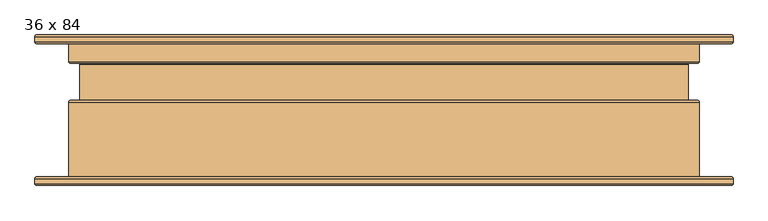
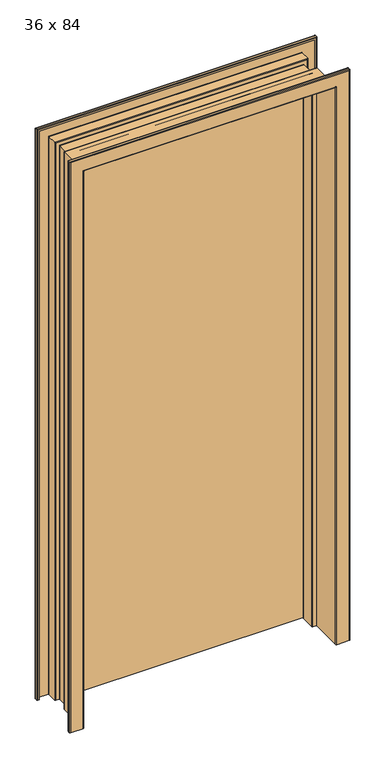
"""IFC4 building model written with IfcOpenShell, lengths in millimetres: door geometry, Door-Dunbarton_Doors-Hollow_Metal_Core : 36 x 84."""

from ifc_helpers import new_model, si_unit, frame, origin, origin_with_axes, place, context, project, spatial, polyline, circle_curve, ellipse_curve, outline, extrude, source, transform, mapped, element, save
from ifc_brep_helpers import plane_surface, cylinder_surface, revolved_surface, advanced_brep


def door_36_x_84_b8b41eee(model_context):
    return source(origin(), model_context, "Body", "SolidModel", [
        advanced_brep(
        [(-505.42825, -96.901, 0.0), (-500.0625, -96.901, 0.0), (-500.0625, -98.45675, 0.0), (-505.42825, -98.45675, 0.0), (-506.44425, -99.47275, 0.0), (-506.44425, -106.9975, 0.0), (-505.42825, -108.0135, 0.0), (-459.77175, -108.0135, 0.0), (-458.75575, -106.9975, 0.0), (-458.75575, 11.65225, 0.0), (-456.184, 14.224, 0.0), (-443.89675, 14.224, 0.0), (-442.88075, 15.24, 0.0), (-442.88075, 67.0306, 0.0), (-443.89675, 68.0466, 0.0), (-456.184, 68.0466, 0.0), (-458.75575, 70.61835, 0.0), (-458.75575, 106.934, 0.0), (-459.77175, 107.95, 0.0), (-505.42825, 107.95, 0.0), (-506.44425, 106.934, 0.0), (-506.44425, 99.40925, 0.0), (-505.42825, 98.39325, 0.0), (-500.0625, 98.39325, 0.0), (-500.0625, 96.8375, 0.0), (-505.42825, 96.8375, 0.0), (-508.0, 99.40925, 0.0), (-508.0, 106.934, 0.0), (-505.42825, 109.50575, 0.0), (-459.77175, 109.50575, 0.0), (-457.2, 106.934, 0.0), (-457.2, 70.61835, 0.0), (-456.184, 69.60235, 0.0), (-443.89675, 69.60235, 0.0), (-441.325, 67.0306, 0.0), (-441.325, 15.24, 0.0), (-443.89675, 12.66825, 0.0), (-456.184, 12.66825, 0.0), (-457.2, 11.65225, 0.0), (-457.2, -106.9975, 0.0), (-459.77175, -109.56925, 0.0), (-505.42825, -109.56925, 0.0), (-508.0, -106.9975, 0.0), (-508.0, -99.47275, 0.0), (-508.0, -99.47275, 2184.4), (-505.42825, -96.901, 2181.82825), (-508.0, -106.9975, 2184.4), (-505.42825, -109.56925, 2181.82825), (-459.77175, -109.56925, 2136.17175), (459.77175, -109.56925, 2136.17175), (459.77175, -109.56925, 0.0), (505.42825, -109.56925, 0.0), (505.42825, -109.56925, 2181.82825), (-457.2, -106.9975, 2133.6), (-457.2, 11.65225, 2133.6), (-456.184, 12.66825, 2132.584), (-443.89675, 12.66825, 2120.29675), (443.89675, 12.66825, 2120.29675), (443.89675, 12.66825, 0.0), (456.184, 12.66825, 0.0), (456.184, 12.66825, 2132.584), (-441.325, 15.24, 2117.725), (-441.325, 67.0306, 2117.725), (-443.89675, 69.60235, 2120.29675), (-456.184, 69.60235, 2132.584), (456.184, 69.60235, 2132.584), (456.184, 69.60235, 0.0), (443.89675, 69.60235, 0.0), (443.89675, 69.60235, 2120.29675), (-457.2, 70.61835, 2133.6), (-457.2, 106.934, 2133.6), (-459.77175, 109.50575, 2136.17175), (-505.42825, 109.50575, 2181.82825), (505.42825, 109.50575, 2181.82825), (505.42825, 109.50575, 0.0), (459.77175, 109.50575, 0.0), (459.77175, 109.50575, 2136.17175), (-508.0, 106.934, 2184.4), (-508.0, 99.40925, 2184.4), (-505.42825, 96.8375, 2181.82825), (-500.0625, 96.8375, 2176.4625), (500.0625, 96.8375, 2176.4625), (500.0625, 96.8375, 0.0), (505.42825, 96.8375, 0.0), (505.42825, 96.8375, 2181.82825), (-500.0625, 98.39325, 2176.4625), (-505.42825, 98.39325, 2181.82825), (505.42825, 98.39325, 2181.82825), (505.42825, 98.39325, 0.0), (500.0625, 98.39325, 0.0), (500.0625, 98.39325, 2176.4625), (-506.44425, 99.40925, 2182.84425), (-506.44425, 106.934, 2182.84425), (-505.42825, 107.95, 2181.82825), (-459.77175, 107.95, 2136.17175), (459.77175, 107.95, 2136.17175), (459.77175, 107.95, 0.0), (505.42825, 107.95, 0.0), (505.42825, 107.95, 2181.82825), (-458.75575, 106.934, 2135.15575), (-458.75575, 70.61835, 2135.15575), (-456.184, 68.0466, 2132.584), (-443.89675, 68.0466, 2120.29675), (443.89675, 68.0466, 2120.29675), (443.89675, 68.0466, 0.0), (456.184, 68.0466, 0.0), (456.184, 68.0466, 2132.584), (-442.88075, 67.0306, 2119.28075), (-442.88075, 15.24, 2119.28075), (-443.89675, 14.224, 2120.29675), (-456.184, 14.224, 2132.584), (456.184, 14.224, 2132.584), (456.184, 14.224, 0.0), (443.89675, 14.224, 0.0), (443.89675, 14.224, 2120.29675), (-458.75575, 11.65225, 2135.15575), (-458.75575, -106.9975, 2135.15575), (-459.77175, -108.0135, 2136.17175), (-505.42825, -108.0135, 2181.82825), (505.42825, -108.0135, 2181.82825), (505.42825, -108.0135, 0.0), (459.77175, -108.0135, 0.0), (459.77175, -108.0135, 2136.17175), (-506.44425, -106.9975, 2182.84425), (-506.44425, -99.47275, 2182.84425), (-505.42825, -98.45675, 2181.82825), (-500.0625, -98.45675, 2176.4625), (500.0625, -98.45675, 2176.4625), (500.0625, -98.45675, 0.0), (505.42825, -98.45675, 0.0), (505.42825, -98.45675, 2181.82825), (-500.0625, -96.901, 2176.4625), (505.42825, -96.901, 2181.82825), (505.42825, -96.901, 0.0), (500.0625, -96.901, 0.0), (500.0625, -96.901, 2176.4625), (508.0, -99.47275, 2184.4), (508.0, -106.9975, 2184.4), (457.2, -106.9975, 2133.6), (457.2, 11.65225, 2133.6), (441.325, 15.24, 2117.725), (441.325, 67.0306, 2117.725), (457.2, 70.61835, 2133.6), (457.2, 106.934, 2133.6), (508.0, 106.934, 2184.4), (508.0, 99.40925, 2184.4), (506.44425, 99.40925, 2182.84425), (506.44425, 106.934, 2182.84425), (458.75575, 106.934, 2135.15575), (458.75575, 70.61835, 2135.15575), (442.88075, 67.0306, 2119.28075), (442.88075, 15.24, 2119.28075), (458.75575, 11.65225, 2135.15575), (458.75575, -106.9975, 2135.15575), (506.44425, -106.9975, 2182.84425), (506.44425, -99.47275, 2182.84425), (508.0, -99.47275, 0.0), (508.0, -106.9975, 0.0), (457.2, -106.9975, 0.0), (457.2, 11.65225, 0.0), (441.325, 15.24, 0.0), (441.325, 67.0306, 0.0), (457.2, 70.61835, 0.0), (457.2, 106.934, 0.0), (508.0, 106.934, 0.0), (508.0, 99.40925, 0.0), (506.44425, 99.40925, 0.0), (506.44425, 106.934, 0.0), (458.75575, 106.934, 0.0), (458.75575, 70.61835, 0.0), (442.88075, 67.0306, 0.0), (442.88075, 15.24, 0.0), (458.75575, 11.65225, 0.0), (458.75575, -106.9975, 0.0), (506.44425, -106.9975, 0.0), (506.44425, -99.47275, 0.0)],
        [
            (0, 1),
            (1, 2),
            (2, 3),
            (3, 4, circle_curve(frame((-505.42825, -99.47275, 0.0), z_axis=(0.0, 0.0, 1.0), x_axis=(0.0, 1.0, 0.0)), 1.016)),
            (4, 5),
            (5, 6, circle_curve(frame((-505.42825, -106.9975, 0.0), z_axis=(0.0, 0.0, 1.0), x_axis=(0.0, 1.0, 0.0)), 1.016)),
            (6, 7),
            (7, 8, circle_curve(frame((-459.77175, -106.9975, 0.0), z_axis=(0.0, 0.0, 1.0), x_axis=(0.0, 1.0, 0.0)), 1.016)),
            (8, 9),
            (9, 10, circle_curve(frame((-456.184, 11.65225, 0.0), z_axis=(0.0, 0.0, -1.0), x_axis=(0.0, 1.0, 0.0)), 2.57175)),
            (10, 11),
            (11, 12, circle_curve(frame((-443.89675, 15.24, 0.0), z_axis=(0.0, 0.0, 1.0), x_axis=(0.0, 1.0, 0.0)), 1.016)),
            (12, 13),
            (13, 14, circle_curve(frame((-443.89675, 67.0306, 0.0), z_axis=(0.0, 0.0, 1.0), x_axis=(0.0, 1.0, 0.0)), 1.016)),
            (14, 15),
            (15, 16, circle_curve(frame((-456.184, 70.61835, 0.0), z_axis=(0.0, 0.0, -1.0), x_axis=(0.0, 1.0, 0.0)), 2.57175)),
            (16, 17),
            (17, 18, circle_curve(frame((-459.77175, 106.934, 0.0), z_axis=(0.0, 0.0, 1.0), x_axis=(0.0, 1.0, 0.0)), 1.016)),
            (18, 19),
            (19, 20, circle_curve(frame((-505.42825, 106.934, 0.0), z_axis=(0.0, 0.0, 1.0), x_axis=(0.0, 1.0, 0.0)), 1.016)),
            (20, 21),
            (21, 22, circle_curve(frame((-505.42825, 99.40925, 0.0), z_axis=(0.0, 0.0, 1.0), x_axis=(0.0, 1.0, 0.0)), 1.016)),
            (22, 23),
            (23, 24),
            (24, 25),
            (25, 26, circle_curve(frame((-505.42825, 99.40925, 0.0), z_axis=(0.0, 0.0, -1.0), x_axis=(0.0, 1.0, 0.0)), 2.57175)),
            (26, 27),
            (27, 28, circle_curve(frame((-505.42825, 106.934, 0.0), z_axis=(0.0, 0.0, -1.0), x_axis=(0.0, 1.0, 0.0)), 2.57175)),
            (28, 29),
            (29, 30, circle_curve(frame((-459.77175, 106.934, 0.0), z_axis=(0.0, 0.0, -1.0), x_axis=(0.0, 1.0, 0.0)), 2.57175)),
            (30, 31),
            (31, 32, circle_curve(frame((-456.184, 70.61835, 0.0), z_axis=(0.0, 0.0, 1.0), x_axis=(0.0, 1.0, 0.0)), 1.016)),
            (32, 33),
            (33, 34, circle_curve(frame((-443.89675, 67.0306, 0.0), z_axis=(0.0, 0.0, -1.0), x_axis=(0.0, 1.0, 0.0)), 2.57175)),
            (34, 35),
            (35, 36, circle_curve(frame((-443.89675, 15.24, 0.0), z_axis=(0.0, 0.0, -1.0), x_axis=(0.0, 1.0, 0.0)), 2.57175)),
            (36, 37),
            (37, 38, circle_curve(frame((-456.184, 11.65225, 0.0), z_axis=(0.0, 0.0, 1.0), x_axis=(0.0, 1.0, 0.0)), 1.016)),
            (38, 39),
            (39, 40, circle_curve(frame((-459.77175, -106.9975, 0.0), z_axis=(0.0, 0.0, -1.0), x_axis=(0.0, 1.0, 0.0)), 2.57175)),
            (40, 41),
            (41, 42, circle_curve(frame((-505.42825, -106.9975, 0.0), z_axis=(0.0, 0.0, -1.0), x_axis=(0.0, 1.0, 0.0)), 2.57175)),
            (42, 43),
            (43, 0, circle_curve(frame((-505.42825, -99.47275, 0.0), z_axis=(0.0, 0.0, -1.0), x_axis=(0.0, 1.0, 0.0)), 2.57175)),
            (43, 44),
            (44, 45, ellipse_curve(frame((-505.42825, -99.47275, 2181.82825), z_axis=(-0.7071067811865475, 0.0, -0.7071067811865475), x_axis=(0.7071067811865474, 0.0, -0.7071067811865476)), 3.6370037, 2.57175)),
            (45, 0),
            (42, 46),
            (46, 44),
            (41, 47),
            (47, 46, ellipse_curve(frame((-505.42825, -106.9975, 2181.82825), z_axis=(-0.7071067811865475, 0.0, -0.7071067811865475), x_axis=(0.7071067811865474, 0.0, -0.7071067811865476)), 3.6370037, 2.57175)),
            (40, 48),
            (48, 49),
            (49, 50),
            (50, 51),
            (51, 52),
            (52, 47),
            (39, 53),
            (53, 48, ellipse_curve(frame((-459.77175, -106.9975, 2136.17175), z_axis=(-0.7071067811865475, 0.0, -0.7071067811865475), x_axis=(0.7071067811865474, 0.0, -0.7071067811865476)), 3.6370037, 2.57175)),
            (38, 54),
            (54, 53),
            (37, 55),
            (55, 54, ellipse_curve(frame((-456.184, 11.65225, 2132.584), z_axis=(0.7071067811865475, 0.0, 0.7071067811865475), x_axis=(-0.7071067811865474, 0.0, 0.7071067811865476)), 1.436841, 1.016)),
            (36, 56),
            (56, 57),
            (57, 58),
            (58, 59),
            (59, 60),
            (60, 55),
            (35, 61),
            (61, 56, ellipse_curve(frame((-443.89675, 15.24, 2120.29675), z_axis=(-0.7071067811865475, 0.0, -0.7071067811865475), x_axis=(0.7071067811865474, 0.0, -0.7071067811865476)), 3.6370037, 2.57175)),
            (34, 62),
            (62, 61),
            (33, 63),
            (63, 62, ellipse_curve(frame((-443.89675, 67.0306, 2120.29675), z_axis=(-0.7071067811865475, 0.0, -0.7071067811865475), x_axis=(0.7071067811865474, 0.0, -0.7071067811865476)), 3.6370037, 2.57175)),
            (32, 64),
            (64, 65),
            (65, 66),
            (66, 67),
            (67, 68),
            (68, 63),
            (31, 69),
            (69, 64, ellipse_curve(frame((-456.184, 70.61835, 2132.584), z_axis=(0.7071067811865475, 0.0, 0.7071067811865475), x_axis=(-0.7071067811865474, 0.0, 0.7071067811865476)), 1.436841, 1.016)),
            (30, 70),
            (70, 69),
            (29, 71),
            (71, 70, ellipse_curve(frame((-459.77175, 106.934, 2136.17175), z_axis=(-0.7071067811865475, 0.0, -0.7071067811865475), x_axis=(0.7071067811865474, 0.0, -0.7071067811865476)), 3.6370037, 2.57175)),
            (28, 72),
            (72, 73),
            (73, 74),
            (74, 75),
            (75, 76),
            (76, 71),
            (27, 77),
            (77, 72, ellipse_curve(frame((-505.42825, 106.934, 2181.82825), z_axis=(-0.7071067811865475, 0.0, -0.7071067811865475), x_axis=(0.7071067811865474, 0.0, -0.7071067811865476)), 3.6370037, 2.57175)),
            (26, 78),
            (78, 77),
            (25, 79),
            (79, 78, ellipse_curve(frame((-505.42825, 99.40925, 2181.82825), z_axis=(-0.7071067811865475, 0.0, -0.7071067811865475), x_axis=(0.7071067811865474, 0.0, -0.7071067811865476)), 3.6370037, 2.57175)),
            (24, 80),
            (80, 81),
            (81, 82),
            (82, 83),
            (83, 84),
            (84, 79),
            (23, 85),
            (85, 80),
            (22, 86),
            (86, 87),
            (87, 88),
            (88, 89),
            (89, 90),
            (90, 85),
            (21, 91),
            (91, 86, ellipse_curve(frame((-505.42825, 99.40925, 2181.82825), z_axis=(0.7071067811865475, 0.0, 0.7071067811865475), x_axis=(-0.7071067811865474, 0.0, 0.7071067811865476)), 1.436841, 1.016)),
            (20, 92),
            (92, 91),
            (19, 93),
            (93, 92, ellipse_curve(frame((-505.42825, 106.934, 2181.82825), z_axis=(0.7071067811865475, 0.0, 0.7071067811865475), x_axis=(-0.7071067811865474, 0.0, 0.7071067811865476)), 1.436841, 1.016)),
            (18, 94),
            (94, 95),
            (95, 96),
            (96, 97),
            (97, 98),
            (98, 93),
            (17, 99),
            (99, 94, ellipse_curve(frame((-459.77175, 106.934, 2136.17175), z_axis=(0.7071067811865475, 0.0, 0.7071067811865475), x_axis=(-0.7071067811865474, 0.0, 0.7071067811865476)), 1.436841, 1.016)),
            (16, 100),
            (100, 99),
            (15, 101),
            (101, 100, ellipse_curve(frame((-456.184, 70.61835, 2132.584), z_axis=(-0.7071067811865475, 0.0, -0.7071067811865475), x_axis=(0.7071067811865474, 0.0, -0.7071067811865476)), 3.6370037, 2.57175)),
            (14, 102),
            (102, 103),
            (103, 104),
            (104, 105),
            (105, 106),
            (106, 101),
            (13, 107),
            (107, 102, ellipse_curve(frame((-443.89675, 67.0306, 2120.29675), z_axis=(0.7071067811865475, 0.0, 0.7071067811865475), x_axis=(-0.7071067811865474, 0.0, 0.7071067811865476)), 1.436841, 1.016)),
            (12, 108),
            (108, 107),
            (11, 109),
            (109, 108, ellipse_curve(frame((-443.89675, 15.24, 2120.29675), z_axis=(0.7071067811865475, 0.0, 0.7071067811865475), x_axis=(-0.7071067811865474, 0.0, 0.7071067811865476)), 1.436841, 1.016)),
            (10, 110),
            (110, 111),
            (111, 112),
            (112, 113),
            (113, 114),
            (114, 109),
            (9, 115),
            (115, 110, ellipse_curve(frame((-456.184, 11.65225, 2132.584), z_axis=(-0.7071067811865475, 0.0, -0.7071067811865475), x_axis=(0.7071067811865474, 0.0, -0.7071067811865476)), 3.6370037, 2.57175)),
            (8, 116),
            (116, 115),
            (7, 117),
            (117, 116, ellipse_curve(frame((-459.77175, -106.9975, 2136.17175), z_axis=(0.7071067811865475, 0.0, 0.7071067811865475), x_axis=(-0.7071067811865474, 0.0, 0.7071067811865476)), 1.436841, 1.016)),
            (6, 118),
            (118, 119),
            (119, 120),
            (120, 121),
            (121, 122),
            (122, 117),
            (5, 123),
            (123, 118, ellipse_curve(frame((-505.42825, -106.9975, 2181.82825), z_axis=(0.7071067811865475, 0.0, 0.7071067811865475), x_axis=(-0.7071067811865474, 0.0, 0.7071067811865476)), 1.436841, 1.016)),
            (4, 124),
            (124, 123),
            (3, 125),
            (125, 124, ellipse_curve(frame((-505.42825, -99.47275, 2181.82825), z_axis=(0.7071067811865475, 0.0, 0.7071067811865475), x_axis=(-0.7071067811865474, 0.0, 0.7071067811865476)), 1.436841, 1.016)),
            (2, 126),
            (126, 127),
            (127, 128),
            (128, 129),
            (129, 130),
            (130, 125),
            (1, 131),
            (131, 126),
            (45, 132),
            (132, 133),
            (133, 134),
            (134, 135),
            (135, 131),
            (44, 136),
            (136, 132, ellipse_curve(frame((505.42825, -99.47275, 2181.82825), z_axis=(-0.7071067811865475, 0.0, 0.7071067811865475), x_axis=(-0.7071067811865476, 0.0, -0.7071067811865474)), 3.6370037, 2.57175)),
            (46, 137),
            (137, 136),
            (52, 137, ellipse_curve(frame((505.42825, -106.9975, 2181.82825), z_axis=(-0.7071067811865475, 0.0, 0.7071067811865475), x_axis=(-0.7071067811865476, 0.0, -0.7071067811865474)), 3.6370037, 2.57175)),
            (53, 138),
            (138, 49, ellipse_curve(frame((459.77175, -106.9975, 2136.17175), z_axis=(-0.7071067811865475, 0.0, 0.7071067811865475), x_axis=(-0.7071067811865476, 0.0, -0.7071067811865474)), 3.6370037, 2.57175)),
            (54, 139),
            (139, 138),
            (60, 139, ellipse_curve(frame((456.184, 11.65225, 2132.584), z_axis=(0.7071067811865475, 0.0, -0.7071067811865475), x_axis=(0.7071067811865476, 0.0, 0.7071067811865474)), 1.436841, 1.016)),
            (61, 140),
            (140, 57, ellipse_curve(frame((443.89675, 15.24, 2120.29675), z_axis=(-0.7071067811865475, 0.0, 0.7071067811865475), x_axis=(-0.7071067811865476, 0.0, -0.7071067811865474)), 3.6370037, 2.57175)),
            (62, 141),
            (141, 140),
            (68, 141, ellipse_curve(frame((443.89675, 67.0306, 2120.29675), z_axis=(-0.7071067811865475, 0.0, 0.7071067811865475), x_axis=(-0.7071067811865476, 0.0, -0.7071067811865474)), 3.6370037, 2.57175)),
            (69, 142),
            (142, 65, ellipse_curve(frame((456.184, 70.61835, 2132.584), z_axis=(0.7071067811865475, 0.0, -0.7071067811865475), x_axis=(0.7071067811865476, 0.0, 0.7071067811865474)), 1.436841, 1.016)),
            (70, 143),
            (143, 142),
            (76, 143, ellipse_curve(frame((459.77175, 106.934, 2136.17175), z_axis=(-0.7071067811865475, 0.0, 0.7071067811865475), x_axis=(-0.7071067811865476, 0.0, -0.7071067811865474)), 3.6370037, 2.57175)),
            (77, 144),
            (144, 73, ellipse_curve(frame((505.42825, 106.934, 2181.82825), z_axis=(-0.7071067811865475, 0.0, 0.7071067811865475), x_axis=(-0.7071067811865476, 0.0, -0.7071067811865474)), 3.6370037, 2.57175)),
            (78, 145),
            (145, 144),
            (84, 145, ellipse_curve(frame((505.42825, 99.40925, 2181.82825), z_axis=(-0.7071067811865475, 0.0, 0.7071067811865475), x_axis=(-0.7071067811865476, 0.0, -0.7071067811865474)), 3.6370037, 2.57175)),
            (90, 81),
            (91, 146),
            (146, 87, ellipse_curve(frame((505.42825, 99.40925, 2181.82825), z_axis=(0.7071067811865475, 0.0, -0.7071067811865475), x_axis=(0.7071067811865476, 0.0, 0.7071067811865474)), 1.436841, 1.016)),
            (92, 147),
            (147, 146),
            (98, 147, ellipse_curve(frame((505.42825, 106.934, 2181.82825), z_axis=(0.7071067811865475, 0.0, -0.7071067811865475), x_axis=(0.7071067811865476, 0.0, 0.7071067811865474)), 1.436841, 1.016)),
            (99, 148),
            (148, 95, ellipse_curve(frame((459.77175, 106.934, 2136.17175), z_axis=(0.7071067811865475, 0.0, -0.7071067811865475), x_axis=(0.7071067811865476, 0.0, 0.7071067811865474)), 1.436841, 1.016)),
            (100, 149),
            (149, 148),
            (106, 149, ellipse_curve(frame((456.184, 70.61835, 2132.584), z_axis=(-0.7071067811865475, 0.0, 0.7071067811865475), x_axis=(-0.7071067811865476, 0.0, -0.7071067811865474)), 3.6370037, 2.57175)),
            (107, 150),
            (150, 103, ellipse_curve(frame((443.89675, 67.0306, 2120.29675), z_axis=(0.7071067811865475, 0.0, -0.7071067811865475), x_axis=(0.7071067811865476, 0.0, 0.7071067811865474)), 1.436841, 1.016)),
            (108, 151),
            (151, 150),
            (114, 151, ellipse_curve(frame((443.89675, 15.24, 2120.29675), z_axis=(0.7071067811865475, 0.0, -0.7071067811865475), x_axis=(0.7071067811865476, 0.0, 0.7071067811865474)), 1.436841, 1.016)),
            (115, 152),
            (152, 111, ellipse_curve(frame((456.184, 11.65225, 2132.584), z_axis=(-0.7071067811865475, 0.0, 0.7071067811865475), x_axis=(-0.7071067811865476, 0.0, -0.7071067811865474)), 3.6370037, 2.57175)),
            (116, 153),
            (153, 152),
            (122, 153, ellipse_curve(frame((459.77175, -106.9975, 2136.17175), z_axis=(0.7071067811865475, 0.0, -0.7071067811865475), x_axis=(0.7071067811865476, 0.0, 0.7071067811865474)), 1.436841, 1.016)),
            (123, 154),
            (154, 119, ellipse_curve(frame((505.42825, -106.9975, 2181.82825), z_axis=(0.7071067811865475, 0.0, -0.7071067811865475), x_axis=(0.7071067811865476, 0.0, 0.7071067811865474)), 1.436841, 1.016)),
            (124, 155),
            (155, 154),
            (130, 155, ellipse_curve(frame((505.42825, -99.47275, 2181.82825), z_axis=(0.7071067811865475, 0.0, -0.7071067811865475), x_axis=(0.7071067811865476, 0.0, 0.7071067811865474)), 1.436841, 1.016)),
            (135, 127),
            (133, 156, circle_curve(frame((505.42825, -99.47275, 0.0), z_axis=(0.0, 0.0, -1.0), x_axis=(0.0, 1.0, 0.0)), 2.57175)),
            (156, 157),
            (157, 51, circle_curve(frame((505.42825, -106.9975, 0.0), z_axis=(0.0, 0.0, -1.0), x_axis=(0.0, 1.0, 0.0)), 2.57175)),
            (50, 158, circle_curve(frame((459.77175, -106.9975, 0.0), z_axis=(0.0, 0.0, -1.0), x_axis=(0.0, 1.0, 0.0)), 2.57175)),
            (158, 159),
            (159, 59, circle_curve(frame((456.184, 11.65225, 0.0), z_axis=(0.0, 0.0, 1.0), x_axis=(0.0, 1.0, 0.0)), 1.016)),
            (58, 160, circle_curve(frame((443.89675, 15.24, 0.0), z_axis=(0.0, 0.0, -1.0), x_axis=(0.0, 1.0, 0.0)), 2.57175)),
            (160, 161),
            (161, 67, circle_curve(frame((443.89675, 67.0306, 0.0), z_axis=(0.0, 0.0, -1.0), x_axis=(0.0, 1.0, 0.0)), 2.57175)),
            (66, 162, circle_curve(frame((456.184, 70.61835, 0.0), z_axis=(0.0, 0.0, 1.0), x_axis=(0.0, 1.0, 0.0)), 1.016)),
            (162, 163),
            (163, 75, circle_curve(frame((459.77175, 106.934, 0.0), z_axis=(0.0, 0.0, -1.0), x_axis=(0.0, 1.0, 0.0)), 2.57175)),
            (74, 164, circle_curve(frame((505.42825, 106.934, 0.0), z_axis=(0.0, 0.0, -1.0), x_axis=(0.0, 1.0, 0.0)), 2.57175)),
            (164, 165),
            (165, 83, circle_curve(frame((505.42825, 99.40925, 0.0), z_axis=(0.0, 0.0, -1.0), x_axis=(0.0, 1.0, 0.0)), 2.57175)),
            (82, 89),
            (88, 166, circle_curve(frame((505.42825, 99.40925, 0.0), z_axis=(0.0, 0.0, 1.0), x_axis=(0.0, 1.0, 0.0)), 1.016)),
            (166, 167),
            (167, 97, circle_curve(frame((505.42825, 106.934, 0.0), z_axis=(0.0, 0.0, 1.0), x_axis=(0.0, 1.0, 0.0)), 1.016)),
            (96, 168, circle_curve(frame((459.77175, 106.934, 0.0), z_axis=(0.0, 0.0, 1.0), x_axis=(0.0, 1.0, 0.0)), 1.016)),
            (168, 169),
            (169, 105, circle_curve(frame((456.184, 70.61835, 0.0), z_axis=(0.0, 0.0, -1.0), x_axis=(0.0, 1.0, 0.0)), 2.57175)),
            (104, 170, circle_curve(frame((443.89675, 67.0306, 0.0), z_axis=(0.0, 0.0, 1.0), x_axis=(0.0, 1.0, 0.0)), 1.016)),
            (170, 171),
            (171, 113, circle_curve(frame((443.89675, 15.24, 0.0), z_axis=(0.0, 0.0, 1.0), x_axis=(0.0, 1.0, 0.0)), 1.016)),
            (112, 172, circle_curve(frame((456.184, 11.65225, 0.0), z_axis=(0.0, 0.0, -1.0), x_axis=(0.0, 1.0, 0.0)), 2.57175)),
            (172, 173),
            (173, 121, circle_curve(frame((459.77175, -106.9975, 0.0), z_axis=(0.0, 0.0, 1.0), x_axis=(0.0, 1.0, 0.0)), 1.016)),
            (120, 174, circle_curve(frame((505.42825, -106.9975, 0.0), z_axis=(0.0, 0.0, 1.0), x_axis=(0.0, 1.0, 0.0)), 1.016)),
            (174, 175),
            (175, 129, circle_curve(frame((505.42825, -99.47275, 0.0), z_axis=(0.0, 0.0, 1.0), x_axis=(0.0, 1.0, 0.0)), 1.016)),
            (128, 134),
            (136, 156),
            (137, 157),
            (138, 158),
            (139, 159),
            (140, 160),
            (141, 161),
            (142, 162),
            (143, 163),
            (144, 164),
            (145, 165),
            (146, 166),
            (147, 167),
            (148, 168),
            (149, 169),
            (150, 170),
            (151, 171),
            (152, 172),
            (153, 173),
            (154, 174),
            (155, 175),
        ],
        [
            plane_surface(frame((-468.3125, 96.8375, 0.0), z_axis=(0.0, 0.0, -1.0), x_axis=(1.0, 0.0, 0.0))),
            cylinder_surface(frame((-505.42825, -99.47275, 0.0), z_axis=(0.0, 0.0, -1.0), x_axis=(0.0, 1.0, 0.0)), 2.57175),
            plane_surface(frame((-508.0, -99.47275, 0.0), z_axis=(-1.0, 0.0, 0.0), x_axis=(0.0, 0.0, 1.0))),
            cylinder_surface(frame((-505.42825, -106.9975, 0.0), z_axis=(0.0, 0.0, -1.0), x_axis=(0.0, 1.0, 0.0)), 2.57175),
            plane_surface(frame((-505.42825, -109.56925, 0.0), z_axis=(0.0, -1.0, 0.0), x_axis=(0.0, 0.0, 1.0))),
            cylinder_surface(frame((-459.77175, -106.9975, 0.0), z_axis=(0.0, 0.0, -1.0), x_axis=(0.0, 1.0, 0.0)), 2.57175),
            plane_surface(frame((-457.2, -106.9975, 0.0), z_axis=(1.0, 0.0, 0.0), x_axis=(0.0, 0.0, 1.0))),
            revolved_surface(polyline([(-456.184, 12.66825, 2133.600000014587), (-456.184, 12.66825, 0.0)]), (-456.184, 11.65225, 0.0), (0.0, 0.0, 1.0)),
            plane_surface(frame((-456.184, 12.66825, 0.0), z_axis=(0.0, -1.0, 0.0), x_axis=(0.0, 0.0, 1.0))),
            cylinder_surface(frame((-443.89675, 15.24, 0.0), z_axis=(0.0, 0.0, -1.0), x_axis=(0.0, 1.0, 0.0)), 2.57175),
            plane_surface(frame((-441.325, 15.24, 0.0), z_axis=(1.0, 0.0, 0.0), x_axis=(0.0, 0.0, 1.0))),
            cylinder_surface(frame((-443.89675, 67.0306, 0.0), z_axis=(0.0, 0.0, -1.0), x_axis=(0.0, 1.0, 0.0)), 2.57175),
            plane_surface(frame((-443.89675, 69.60235, 0.0), z_axis=(0.0, 1.0, 0.0), x_axis=(0.0, 0.0, 1.0))),
            revolved_surface(polyline([(-456.184, 71.63435000000001, 2133.600000014587), (-456.184, 71.63435000000001, 0.0)]), (-456.184, 70.61835, 0.0), (0.0, 0.0, 1.0)),
            plane_surface(frame((-457.2, 70.61835, 0.0), z_axis=(1.0, 0.0, 0.0), x_axis=(0.0, 0.0, 1.0))),
            cylinder_surface(frame((-459.77175, 106.934, 0.0), z_axis=(0.0, 0.0, -1.0), x_axis=(0.0, 1.0, 0.0)), 2.57175),
            plane_surface(frame((-459.77175, 109.50575, 0.0), z_axis=(0.0, 1.0, 0.0), x_axis=(0.0, 0.0, 1.0))),
            cylinder_surface(frame((-505.42825, 106.934, 0.0), z_axis=(0.0, 0.0, -1.0), x_axis=(0.0, 1.0, 0.0)), 2.57175),
            plane_surface(frame((-508.0, 106.934, 0.0), z_axis=(-1.0, 0.0, 0.0), x_axis=(0.0, 0.0, 1.0))),
            cylinder_surface(frame((-505.42825, 99.40925, 0.0), z_axis=(0.0, 0.0, -1.0), x_axis=(0.0, 1.0, 0.0)), 2.57175),
            plane_surface(frame((-505.42825, 96.8375, 0.0), z_axis=(0.0, -1.0, 0.0), x_axis=(0.0, 0.0, 1.0))),
            plane_surface(frame((-500.0625, 96.8375, 0.0), z_axis=(1.0, 0.0, 0.0), x_axis=(0.0, 0.0, 1.0))),
            plane_surface(frame((-500.0625, 98.39325, 0.0), z_axis=(0.0, 1.0, 0.0), x_axis=(0.0, 0.0, 1.0))),
            revolved_surface(polyline([(-505.42825, 100.42525, 2182.844250014587), (-505.42825, 100.42525, 0.0)]), (-505.42825, 99.40925, 0.0), (0.0, 0.0, 1.0)),
            plane_surface(frame((-506.44425, 99.40925, 0.0), z_axis=(1.0, 0.0, 0.0), x_axis=(0.0, 0.0, 1.0))),
            revolved_surface(polyline([(-505.42825, 107.95, 2182.844250014587), (-505.42825, 107.95, 0.0)]), (-505.42825, 106.934, 0.0), (0.0, 0.0, 1.0)),
            plane_surface(frame((-505.42825, 107.95, 0.0), z_axis=(0.0, -1.0, 0.0), x_axis=(0.0, 0.0, 1.0))),
            revolved_surface(polyline([(-459.77175, 107.95, 2137.187750014587), (-459.77175, 107.95, 0.0)]), (-459.77175, 106.934, 0.0), (0.0, 0.0, 1.0)),
            plane_surface(frame((-458.75575, 106.934, 0.0), z_axis=(-1.0, 0.0, 0.0), x_axis=(0.0, 0.0, 1.0))),
            cylinder_surface(frame((-456.184, 70.61835, 0.0), z_axis=(0.0, 0.0, -1.0), x_axis=(0.0, 1.0, 0.0)), 2.57175),
            plane_surface(frame((-456.184, 68.0466, 0.0), z_axis=(0.0, -1.0, 0.0), x_axis=(0.0, 0.0, 1.0))),
            revolved_surface(polyline([(-443.89675, 68.04660000000001, 2121.312750014587), (-443.89675, 68.04660000000001, 0.0)]), (-443.89675, 67.0306, 0.0), (0.0, 0.0, 1.0)),
            plane_surface(frame((-442.88075, 67.0306, 0.0), z_axis=(-1.0, 0.0, 0.0), x_axis=(0.0, 0.0, 1.0))),
            revolved_surface(polyline([(-443.89675, 16.256, 2121.312750014587), (-443.89675, 16.256, 0.0)]), (-443.89675, 15.24, 0.0), (0.0, 0.0, 1.0)),
            plane_surface(frame((-443.89675, 14.224, 0.0), z_axis=(0.0, 1.0, 0.0), x_axis=(0.0, 0.0, 1.0))),
            cylinder_surface(frame((-456.184, 11.65225, 0.0), z_axis=(0.0, 0.0, -1.0), x_axis=(0.0, 1.0, 0.0)), 2.57175),
            plane_surface(frame((-458.75575, 11.65225, 0.0), z_axis=(-1.0, 0.0, 0.0), x_axis=(0.0, 0.0, 1.0))),
            revolved_surface(polyline([(-459.77175, -105.9815, 2137.187750014587), (-459.77175, -105.9815, 0.0)]), (-459.77175, -106.9975, 0.0), (0.0, 0.0, 1.0)),
            plane_surface(frame((-459.77175, -108.0135, 0.0), z_axis=(0.0, 1.0, 0.0), x_axis=(0.0, 0.0, 1.0))),
            revolved_surface(polyline([(-505.42825, -105.9815, 2182.844250014587), (-505.42825, -105.9815, 0.0)]), (-505.42825, -106.9975, 0.0), (0.0, 0.0, 1.0)),
            plane_surface(frame((-506.44425, -106.9975, 0.0), z_axis=(1.0, 0.0, 0.0), x_axis=(0.0, 0.0, 1.0))),
            revolved_surface(polyline([(-505.42825, -98.45675, 2182.844250014587), (-505.42825, -98.45675, 0.0)]), (-505.42825, -99.47275, 0.0), (0.0, 0.0, 1.0)),
            plane_surface(frame((-505.42825, -98.45675, 0.0), z_axis=(0.0, -1.0, 0.0), x_axis=(0.0, 0.0, 1.0))),
            plane_surface(frame((-500.0625, -98.45675, 0.0), z_axis=(1.0, 0.0, 0.0), x_axis=(0.0, 0.0, 1.0))),
            plane_surface(frame((-500.0625, -96.901, 0.0), z_axis=(0.0, 1.0, 0.0), x_axis=(0.0, 0.0, 1.0))),
            cylinder_surface(frame((-468.3125, -99.47275, 2181.82825), z_axis=(-1.0, 0.0, 0.0), x_axis=(0.0, 1.0, 0.0)), 2.57175),
            plane_surface(frame((-508.0, -99.47275, 2184.4), z_axis=(0.0, 0.0, 1.0), x_axis=(1.0, 0.0, 0.0))),
            cylinder_surface(frame((-468.3125, -106.9975, 2181.82825), z_axis=(-1.0, 0.0, 0.0), x_axis=(0.0, 1.0, 0.0)), 2.57175),
            cylinder_surface(frame((-468.3125, -106.9975, 2136.17175), z_axis=(-1.0, 0.0, 0.0), x_axis=(0.0, 1.0, 0.0)), 2.57175),
            plane_surface(frame((-457.2, -106.9975, 2133.6), z_axis=(0.0, 0.0, -1.0), x_axis=(1.0, 0.0, 0.0))),
            revolved_surface(polyline([(457.20000001458686, 12.66825, 2132.584), (-457.20000001458686, 12.66825, 2132.584)]), (-468.3125, 11.65225, 2132.584), (1.0, 0.0, 0.0)),
            cylinder_surface(frame((-468.3125, 15.24, 2120.29675), z_axis=(-1.0, 0.0, 0.0), x_axis=(0.0, 1.0, 0.0)), 2.57175),
            plane_surface(frame((-441.325, 15.24, 2117.725), z_axis=(0.0, 0.0, -1.0), x_axis=(1.0, 0.0, 0.0))),
            cylinder_surface(frame((-468.3125, 67.0306, 2120.29675), z_axis=(-1.0, 0.0, 0.0), x_axis=(0.0, 1.0, 0.0)), 2.57175),
            revolved_surface(polyline([(457.20000001458686, 71.63435000000001, 2132.584), (-457.20000001458686, 71.63435000000001, 2132.584)]), (-468.3125, 70.61835, 2132.584), (1.0, 0.0, 0.0)),
            plane_surface(frame((-457.2, 70.61835, 2133.6), z_axis=(0.0, 0.0, -1.0), x_axis=(1.0, 0.0, 0.0))),
            cylinder_surface(frame((-468.3125, 106.934, 2136.17175), z_axis=(-1.0, 0.0, 0.0), x_axis=(0.0, 1.0, 0.0)), 2.57175),
            cylinder_surface(frame((-468.3125, 106.934, 2181.82825), z_axis=(-1.0, 0.0, 0.0), x_axis=(0.0, 1.0, 0.0)), 2.57175),
            plane_surface(frame((-508.0, 106.934, 2184.4), z_axis=(0.0, 0.0, 1.0), x_axis=(1.0, 0.0, 0.0))),
            cylinder_surface(frame((-468.3125, 99.40925, 2181.82825), z_axis=(-1.0, 0.0, 0.0), x_axis=(0.0, 1.0, 0.0)), 2.57175),
            plane_surface(frame((-500.0625, 96.8375, 2176.4625), z_axis=(0.0, 0.0, -1.0), x_axis=(1.0, 0.0, 0.0))),
            revolved_surface(polyline([(506.4442500145868, 100.42525, 2181.82825), (-506.4442500145868, 100.42525, 2181.82825)]), (-468.3125, 99.40925, 2181.82825), (1.0, 0.0, 0.0)),
            plane_surface(frame((-506.44425, 99.40925, 2182.84425), z_axis=(0.0, 0.0, -1.0), x_axis=(1.0, 0.0, 0.0))),
            revolved_surface(polyline([(506.4442500145868, 107.95, 2181.82825), (-506.4442500145868, 107.95, 2181.82825)]), (-468.3125, 106.934, 2181.82825), (1.0, 0.0, 0.0)),
            revolved_surface(polyline([(460.7877500145869, 107.95, 2136.17175), (-460.78775001458683, 107.95, 2136.17175)]), (-468.3125, 106.934, 2136.17175), (1.0, 0.0, 0.0)),
            plane_surface(frame((-458.75575, 106.934, 2135.15575), z_axis=(0.0, 0.0, 1.0), x_axis=(1.0, 0.0, 0.0))),
            cylinder_surface(frame((-468.3125, 70.61835, 2132.584), z_axis=(-1.0, 0.0, 0.0), x_axis=(0.0, 1.0, 0.0)), 2.57175),
            revolved_surface(polyline([(444.9127500145869, 68.04660000000001, 2120.29675), (-444.91275001458683, 68.04660000000001, 2120.29675)]), (-468.3125, 67.0306, 2120.29675), (1.0, 0.0, 0.0)),
            plane_surface(frame((-442.88075, 67.0306, 2119.28075), z_axis=(0.0, 0.0, 1.0), x_axis=(1.0, 0.0, 0.0))),
            revolved_surface(polyline([(444.9127500145869, 16.256, 2120.29675), (-444.91275001458683, 16.256, 2120.29675)]), (-468.3125, 15.24, 2120.29675), (1.0, 0.0, 0.0)),
            cylinder_surface(frame((-468.3125, 11.65225, 2132.584), z_axis=(-1.0, 0.0, 0.0), x_axis=(0.0, 1.0, 0.0)), 2.57175),
            plane_surface(frame((-458.75575, 11.65225, 2135.15575), z_axis=(0.0, 0.0, 1.0), x_axis=(1.0, 0.0, 0.0))),
            revolved_surface(polyline([(460.7877500145869, -105.9815, 2136.17175), (-460.78775001458683, -105.9815, 2136.17175)]), (-468.3125, -106.9975, 2136.17175), (1.0, 0.0, 0.0)),
            revolved_surface(polyline([(506.4442500145868, -105.9815, 2181.82825), (-506.4442500145868, -105.9815, 2181.82825)]), (-468.3125, -106.9975, 2181.82825), (1.0, 0.0, 0.0)),
            plane_surface(frame((-506.44425, -106.9975, 2182.84425), z_axis=(0.0, 0.0, -1.0), x_axis=(1.0, 0.0, 0.0))),
            revolved_surface(polyline([(506.4442500145868, -98.45675, 2181.82825), (-506.4442500145868, -98.45675, 2181.82825)]), (-468.3125, -99.47275, 2181.82825), (1.0, 0.0, 0.0)),
            plane_surface(frame((-500.0625, -98.45675, 2176.4625), z_axis=(0.0, 0.0, -1.0), x_axis=(1.0, 0.0, 0.0))),
            plane_surface(frame((468.3125, 96.8375, 0.0), z_axis=(0.0, 0.0, -1.0), x_axis=(-1.0, 0.0, 0.0))),
            cylinder_surface(frame((505.42825, -99.47275, 2144.7125), z_axis=(0.0, 0.0, 1.0), x_axis=(0.0, 1.0, 0.0)), 2.57175),
            plane_surface(frame((508.0, -99.47275, 2184.4), z_axis=(1.0, 0.0, 0.0), x_axis=(0.0, 0.0, -1.0))),
            cylinder_surface(frame((505.42825, -106.9975, 2144.7125), z_axis=(0.0, 0.0, 1.0), x_axis=(0.0, 1.0, 0.0)), 2.57175),
            cylinder_surface(frame((459.77175, -106.9975, 2144.7125), z_axis=(0.0, 0.0, 1.0), x_axis=(0.0, 1.0, 0.0)), 2.57175),
            plane_surface(frame((457.2, -106.9975, 2133.6), z_axis=(-1.0, 0.0, 0.0), x_axis=(0.0, 0.0, -1.0))),
            revolved_surface(polyline([(456.184, 12.66825, 0.0), (456.184, 12.66825, 2133.600000014587)]), (456.184, 11.65225, 2144.7125), (0.0, 0.0, -1.0)),
            cylinder_surface(frame((443.89675, 15.24, 2144.7125), z_axis=(0.0, 0.0, 1.0), x_axis=(0.0, 1.0, 0.0)), 2.57175),
            plane_surface(frame((441.325, 15.24, 2117.725), z_axis=(-1.0, 0.0, 0.0), x_axis=(0.0, 0.0, -1.0))),
            cylinder_surface(frame((443.89675, 67.0306, 2144.7125), z_axis=(0.0, 0.0, 1.0), x_axis=(0.0, 1.0, 0.0)), 2.57175),
            revolved_surface(polyline([(456.184, 71.63435000000001, 0.0), (456.184, 71.63435000000001, 2133.600000014587)]), (456.184, 70.61835, 2144.7125), (0.0, 0.0, -1.0)),
            plane_surface(frame((457.2, 70.61835, 2133.6), z_axis=(-1.0, 0.0, 0.0), x_axis=(0.0, 0.0, -1.0))),
            cylinder_surface(frame((459.77175, 106.934, 2144.7125), z_axis=(0.0, 0.0, 1.0), x_axis=(0.0, 1.0, 0.0)), 2.57175),
            cylinder_surface(frame((505.42825, 106.934, 2144.7125), z_axis=(0.0, 0.0, 1.0), x_axis=(0.0, 1.0, 0.0)), 2.57175),
            plane_surface(frame((508.0, 106.934, 2184.4), z_axis=(1.0, 0.0, 0.0), x_axis=(0.0, 0.0, -1.0))),
            cylinder_surface(frame((505.42825, 99.40925, 2144.7125), z_axis=(0.0, 0.0, 1.0), x_axis=(0.0, 1.0, 0.0)), 2.57175),
            plane_surface(frame((500.0625, 96.8375, 2176.4625), z_axis=(-1.0, 0.0, 0.0), x_axis=(0.0, 0.0, -1.0))),
            revolved_surface(polyline([(505.42825, 100.42525, 0.0), (505.42825, 100.42525, 2182.844250014587)]), (505.42825, 99.40925, 2144.7125), (0.0, 0.0, -1.0)),
            plane_surface(frame((506.44425, 99.40925, 2182.84425), z_axis=(-1.0, 0.0, 0.0), x_axis=(0.0, 0.0, -1.0))),
            revolved_surface(polyline([(505.42825, 107.95, 0.0), (505.42825, 107.95, 2182.844250014587)]), (505.42825, 106.934, 2144.7125), (0.0, 0.0, -1.0)),
            revolved_surface(polyline([(459.77175, 107.95, 0.0), (459.77175, 107.95, 2137.187750014587)]), (459.77175, 106.934, 2144.7125), (0.0, 0.0, -1.0)),
            plane_surface(frame((458.75575, 106.934, 2135.15575), z_axis=(1.0, 0.0, 0.0), x_axis=(0.0, 0.0, -1.0))),
            cylinder_surface(frame((456.184, 70.61835, 2144.7125), z_axis=(0.0, 0.0, 1.0), x_axis=(0.0, 1.0, 0.0)), 2.57175),
            revolved_surface(polyline([(443.89675, 68.04660000000001, 0.0), (443.89675, 68.04660000000001, 2121.312750014587)]), (443.89675, 67.0306, 2144.7125), (0.0, 0.0, -1.0)),
            plane_surface(frame((442.88075, 67.0306, 2119.28075), z_axis=(1.0, 0.0, 0.0), x_axis=(0.0, 0.0, -1.0))),
            revolved_surface(polyline([(443.89675, 16.256, 0.0), (443.89675, 16.256, 2121.312750014587)]), (443.89675, 15.24, 2144.7125), (0.0, 0.0, -1.0)),
            cylinder_surface(frame((456.184, 11.65225, 2144.7125), z_axis=(0.0, 0.0, 1.0), x_axis=(0.0, 1.0, 0.0)), 2.57175),
            plane_surface(frame((458.75575, 11.65225, 2135.15575), z_axis=(1.0, 0.0, 0.0), x_axis=(0.0, 0.0, -1.0))),
            revolved_surface(polyline([(459.77175, -105.9815, 0.0), (459.77175, -105.9815, 2137.187750014587)]), (459.77175, -106.9975, 2144.7125), (0.0, 0.0, -1.0)),
            revolved_surface(polyline([(505.42825, -105.9815, 0.0), (505.42825, -105.9815, 2182.844250014587)]), (505.42825, -106.9975, 2144.7125), (0.0, 0.0, -1.0)),
            plane_surface(frame((506.44425, -106.9975, 2182.84425), z_axis=(-1.0, 0.0, 0.0), x_axis=(0.0, 0.0, -1.0))),
            revolved_surface(polyline([(505.42825, -98.45675, 0.0), (505.42825, -98.45675, 2182.844250014587)]), (505.42825, -99.47275, 2144.7125), (0.0, 0.0, -1.0)),
            plane_surface(frame((500.0625, -98.45675, 2176.4625), z_axis=(-1.0, 0.0, 0.0), x_axis=(0.0, 0.0, -1.0))),
        ],
        [
            (0, [[1, 2, 3, 4, 5, 6, 7, 8, 9, 10, 11, 12, 13, 14, 15, 16, 17, 18, 19, 20, 21, 22, 23, 24, 25, 26, 27, 28, 29, 30, 31, 32, 33, 34, 35, 36, 37, 38, 39, 40, 41, 42, 43, 44]]),
            (1, [[45, 46, 47, -44]]),
            (2, [[48, 49, -45, -43]]),
            (3, [[50, 51, -48, -42]]),
            (4, [[52, 53, 54, 55, 56, 57, -50, -41]]),
            (5, [[58, 59, -52, -40]]),
            (6, [[60, 61, -58, -39]]),
            (7, [[62, 63, -60, -38]]),
            (8, [[64, 65, 66, 67, 68, 69, -62, -37]]),
            (9, [[70, 71, -64, -36]]),
            (10, [[72, 73, -70, -35]]),
            (11, [[74, 75, -72, -34]]),
            (12, [[76, 77, 78, 79, 80, 81, -74, -33]]),
            (13, [[82, 83, -76, -32]]),
            (14, [[84, 85, -82, -31]]),
            (15, [[86, 87, -84, -30]]),
            (16, [[88, 89, 90, 91, 92, 93, -86, -29]]),
            (17, [[94, 95, -88, -28]]),
            (18, [[96, 97, -94, -27]]),
            (19, [[98, 99, -96, -26]]),
            (20, [[100, 101, 102, 103, 104, 105, -98, -25]]),
            (21, [[106, 107, -100, -24]]),
            (22, [[108, 109, 110, 111, 112, 113, -106, -23]]),
            (23, [[114, 115, -108, -22]]),
            (24, [[116, 117, -114, -21]]),
            (25, [[118, 119, -116, -20]]),
            (26, [[120, 121, 122, 123, 124, 125, -118, -19]]),
            (27, [[126, 127, -120, -18]]),
            (28, [[128, 129, -126, -17]]),
            (29, [[130, 131, -128, -16]]),
            (30, [[132, 133, 134, 135, 136, 137, -130, -15]]),
            (31, [[138, 139, -132, -14]]),
            (32, [[140, 141, -138, -13]]),
            (33, [[142, 143, -140, -12]]),
            (34, [[144, 145, 146, 147, 148, 149, -142, -11]]),
            (35, [[150, 151, -144, -10]]),
            (36, [[152, 153, -150, -9]]),
            (37, [[154, 155, -152, -8]]),
            (38, [[156, 157, 158, 159, 160, 161, -154, -7]]),
            (39, [[162, 163, -156, -6]]),
            (40, [[164, 165, -162, -5]]),
            (41, [[166, 167, -164, -4]]),
            (42, [[168, 169, 170, 171, 172, 173, -166, -3]]),
            (43, [[174, 175, -168, -2]]),
            (44, [[-47, 176, 177, 178, 179, 180, -174, -1]]),
            (45, [[181, 182, -176, -46]]),
            (46, [[183, 184, -181, -49]]),
            (47, [[-57, 185, -183, -51]]),
            (48, [[186, 187, -53, -59]]),
            (49, [[188, 189, -186, -61]]),
            (50, [[-69, 190, -188, -63]]),
            (51, [[191, 192, -65, -71]]),
            (52, [[193, 194, -191, -73]]),
            (53, [[-81, 195, -193, -75]]),
            (54, [[196, 197, -77, -83]]),
            (55, [[198, 199, -196, -85]]),
            (56, [[-93, 200, -198, -87]]),
            (57, [[201, 202, -89, -95]]),
            (58, [[203, 204, -201, -97]]),
            (59, [[-105, 205, -203, -99]]),
            (60, [[-113, 206, -101, -107]]),
            (61, [[207, 208, -109, -115]]),
            (62, [[209, 210, -207, -117]]),
            (63, [[-125, 211, -209, -119]]),
            (64, [[212, 213, -121, -127]]),
            (65, [[214, 215, -212, -129]]),
            (66, [[-137, 216, -214, -131]]),
            (67, [[217, 218, -133, -139]]),
            (68, [[219, 220, -217, -141]]),
            (69, [[-149, 221, -219, -143]]),
            (70, [[222, 223, -145, -151]]),
            (71, [[224, 225, -222, -153]]),
            (72, [[-161, 226, -224, -155]]),
            (73, [[227, 228, -157, -163]]),
            (74, [[229, 230, -227, -165]]),
            (75, [[-173, 231, -229, -167]]),
            (76, [[-180, 232, -169, -175]]),
            (77, [[233, 234, 235, -55, 236, 237, 238, -67, 239, 240, 241, -79, 242, 243, 244, -91, 245, 246, 247, -103, 248, -111, 249, 250, 251, -123, 252, 253, 254, -135, 255, 256, 257, -147, 258, 259, 260, -159, 261, 262, 263, -171, 264, -178]]),
            (78, [[265, -233, -177, -182]]),
            (79, [[266, -234, -265, -184]]),
            (80, [[-56, -235, -266, -185]]),
            (81, [[267, -236, -54, -187]]),
            (82, [[268, -237, -267, -189]]),
            (83, [[-68, -238, -268, -190]]),
            (84, [[269, -239, -66, -192]]),
            (85, [[270, -240, -269, -194]]),
            (86, [[-80, -241, -270, -195]]),
            (87, [[271, -242, -78, -197]]),
            (88, [[272, -243, -271, -199]]),
            (89, [[-92, -244, -272, -200]]),
            (90, [[273, -245, -90, -202]]),
            (91, [[274, -246, -273, -204]]),
            (92, [[-104, -247, -274, -205]]),
            (93, [[-112, -248, -102, -206]]),
            (94, [[275, -249, -110, -208]]),
            (95, [[276, -250, -275, -210]]),
            (96, [[-124, -251, -276, -211]]),
            (97, [[277, -252, -122, -213]]),
            (98, [[278, -253, -277, -215]]),
            (99, [[-136, -254, -278, -216]]),
            (100, [[279, -255, -134, -218]]),
            (101, [[280, -256, -279, -220]]),
            (102, [[-148, -257, -280, -221]]),
            (103, [[281, -258, -146, -223]]),
            (104, [[282, -259, -281, -225]]),
            (105, [[-160, -260, -282, -226]]),
            (106, [[283, -261, -158, -228]]),
            (107, [[284, -262, -283, -230]]),
            (108, [[-172, -263, -284, -231]]),
            (109, [[-179, -264, -170, -232]]),
        ],
    ),
        extrude(outline(polyline([(455.64425, 70.61835), (-455.64425, 70.61835), (-455.64425, 96.8375), (455.64425, 96.8375), (455.64425, 70.61835)])), origin_with_axes(), (0.0, 0.0, 1.0), 2133.6),
    ])


if __name__ == "__main__":
    model = new_model("IFC4")
    model_context = context("Model", 3, world=origin())
    ifc_project = project(units=[si_unit("LENGTHUNIT", "METRE", prefix="MILLI")], contexts=[model_context])
    site = spatial("IfcSite", under=ifc_project)
    building = spatial("IfcBuilding", under=site)
    placement = place(None, origin())
    door_36_x_84_shape = door_36_x_84_b8b41eee(model_context)
    element("IfcDoor", 1, ObjectType="Door-Dunbarton_Doors-Hollow_Metal_Core : 36 x 84", at=placement, inside=building, context=model_context, shape_type="MappedRepresentation", body=[
        mapped(door_36_x_84_shape, transform((0.0, 0.0, 0.0), x_axis=(1.0, 0.0, 0.0), y_axis=(0.0, 1.0, 0.0), z_axis=(0.0, 0.0, 1.0))),
    ])
    save(model, "model.ifc")

# Revit data of these elements
# Type "Door-Dunbarton_Doors-Hollow_Metal_Core : 36 x 84"
#   Type Mark = "15"
#   URL = "http://dunbarton.com/"
#   Product Page URL = "http://dunbarton.com/products/rediframe-door-frames/rediframe-hollow-metal/"
#   Product Name = "Hollow Metal Non Kerfed"
#   Product Documentation Link = "http://dunbarton.com/products/rediframe-door-frames/rediframe-drawings-overview/"
#   Model = "Non-Kerfed"
#   Material = ""
#   Manufacturer = "Dunbarton Corporation"
#   Description = "Hollow Metal Non-Kerfed Profile"
#   Frame Projection Ext. = 0' - 1"
#   Frame Projection Int. = 0' - 1"
#   Frame Width = 0' - 3"
#   Height = 7' - 0"
#   Width = 3' - 0"
#   Non-Kerfed = yes
#   Kerfed = no
#   Hollow Metal Casing = Metal-Dunbarton_Doors-White
#   Flush Door = Metal-Dunbarton_Doors-Aluminum
#   Function = (empty or 0)
#   Wall Closure = (empty or 0)
# Element 1 (IfcDoor, "Door-Dunbarton_Doors-Hollow_Metal_Core : 36 x 84")
#   Materials on its faces: "Metal-Dunbarton_Doors-White", "Metal-Dunbarton_Doors-Aluminum"
# Materials
#   "Metal-Dunbarton_Doors-White": class "Miscellaneous", colour RGB 230 233 236, transparency 0
#   "Metal-Dunbarton_Doors-Aluminum": class "System", colour RGB 143 142 141, transparency 0
